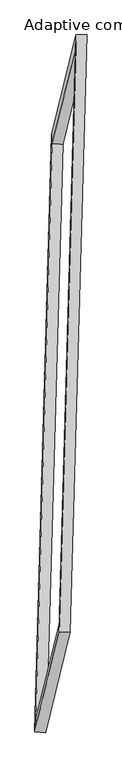
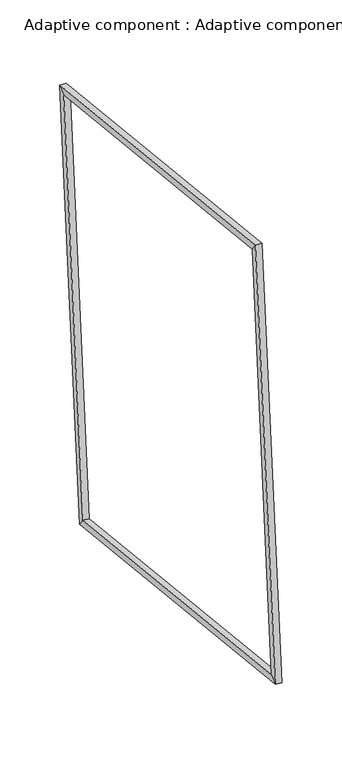
"""IFC4 building model written with IfcOpenShell, lengths in millimetres: proxy geometry, Adaptive component : Adaptive component."""

from ifc_helpers import new_model, si_unit, origin, place, context, project, spatial, faceted_brep, source, transform, mapped, element, save


def adaptive_component_adaptive_component_9e281c95(model_context):
    return source(origin(), model_context, "Body", "Brep", [
        faceted_brep([(102.8835415, 1677.2617731, 3217.8258375), (167.9065869, 1677.1466528, 3217.4014341), (20.8818831, 1075.807039, -1040.1027847), (-44.0190937, 1076.4214269, -1036.1435498), (100.6084864, 1603.8190886, 3162.6188957), (-41.8532434, 1021.1423045, -962.751875), (165.6315318, 1603.7039683, 3162.1944924), (23.0477334, 1020.5279166, -966.71111), (-81.9429645, -2519.8600095, -528.6917056), (-146.7428514, -2515.7106258, -525.2352524), (-140.8993116, -2442.3851611, -470.134985), (-76.0994246, -2446.5345448, -473.5914382), (65.0817393, -1918.5203957, 3728.8125133), (0.1597838, -1914.8702797, 3728.7341349), (1.5624182, -1859.7083771, 3655.2357858), (66.4843738, -1863.3584931, 3655.3141642)], [[[0, 1, 2, 3]], [[4, 0, 3, 5]], [[6, 4, 5, 7]], [[1, 6, 7, 2]], [[3, 2, 8, 9]], [[5, 3, 9, 10]], [[7, 5, 10, 11]], [[2, 7, 11, 8]], [[9, 8, 12, 13]], [[10, 9, 13, 14]], [[11, 10, 14, 15]], [[8, 11, 15, 12]], [[13, 12, 1, 0]], [[14, 13, 0, 4]], [[15, 14, 4, 6]], [[12, 15, 6, 1]]]),
    ])


if __name__ == "__main__":
    model = new_model("IFC4")
    model_context = context("Model", 3, world=origin())
    ifc_project = project(units=[si_unit("LENGTHUNIT", "METRE", prefix="MILLI")], contexts=[model_context])
    site = spatial("IfcSite", under=ifc_project)
    building = spatial("IfcBuilding", under=site)
    placement = place(None, origin())
    adaptive_component_adaptive_component_shape = adaptive_component_adaptive_component_9e281c95(model_context)
    element("IfcBuildingElementProxy", 1, Name="Adaptive component : Adaptive component", ObjectType="Adaptive component : Adaptive component", at=placement, inside=building, context=model_context, shape_type="MappedRepresentation", body=[
        mapped(adaptive_component_adaptive_component_shape, transform((0.0, 0.0, 0.0), x_axis=(1.0, 0.0, 0.0), y_axis=(0.0, 1.0, 0.0), z_axis=(0.0, 0.0, 1.0))),
    ])
    save(model, "model.ifc")

# Revit data of these elements
# Type "Adaptive component : Adaptive component"
#   r [instance default] = 2063.125 mm
#   2r [instance default] = 4126.251 mm
#   Number [instance default] = 5
#   Default Elevation = 0
# Element 1 (IfcBuildingElementProxy, "Adaptive component : Adaptive component")
#   r = 2721.685 mm
#   2r = 5443.37 mm
#   Number = 28
